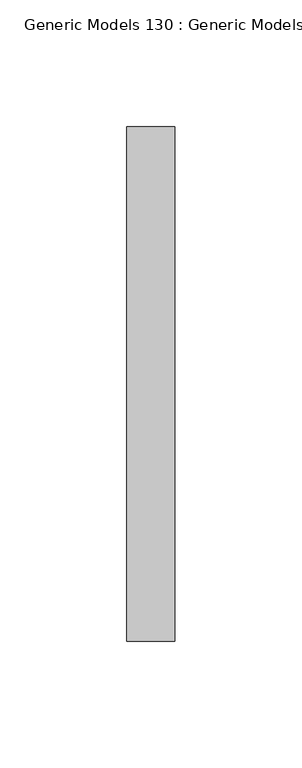
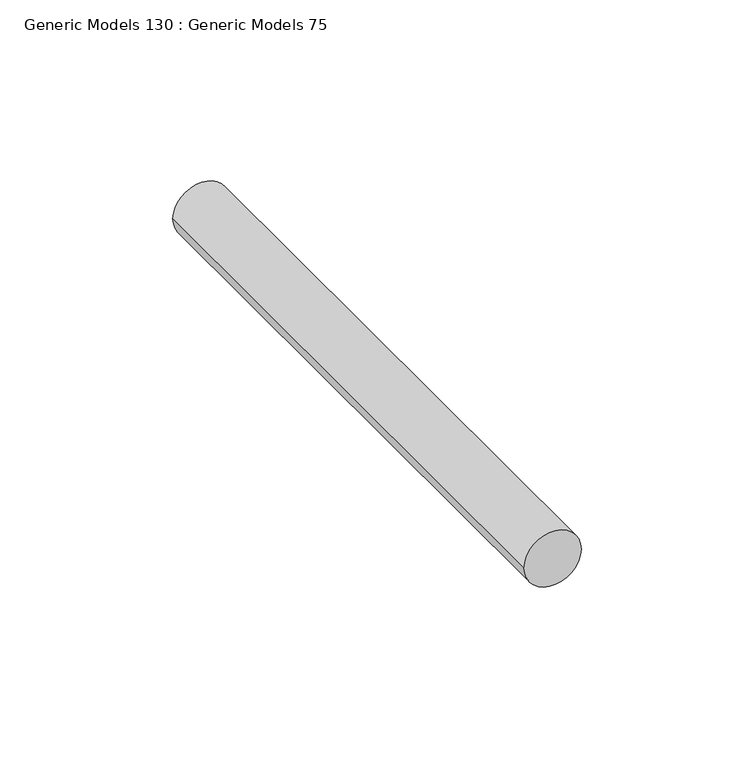
"""IFC4 building model written with IfcOpenShell, lengths in millimetres: proxy geometry, Generic Models 130 : Generic Models 75."""

from ifc_helpers import new_model, si_unit, point, frame, frame_2d, origin, place, context, project, spatial, circle_curve, trimmed, segment, composite_curve, outline, extrude, source, transform, mapped, element, save


def generic_models_130_generic_models_75_e1c93d45(model_context):
    return source(origin(), model_context, "Body", "SweptSolid", [
        extrude(outline(composite_curve([segment(trimmed(circle_curve(frame_2d((268495.4625, 31975.4096032)), 9.525), [point((268495.4625, 31965.8846032))], [point((268495.4625, 31984.9346032))], False, "CARTESIAN"), True, "CONTINUOUS"), segment(trimmed(circle_curve(frame_2d((268495.4625, 31975.4096032)), 9.525), [point((268495.4625, 31984.9346032))], [point((268495.4625, 31965.8846032))], False, "CARTESIAN"), True, "CONTINUOUS")], self_intersect=False)), frame((0.0, 33973.9898424, 0.0), z_axis=(0.0, 1.0, 0.0), x_axis=(0.0, 0.0, 1.0)), (0.0, 0.0, 1.0), 203.2),
    ])


if __name__ == "__main__":
    model = new_model("IFC4")
    model_context = context("Model", 3, world=origin())
    ifc_project = project(units=[si_unit("LENGTHUNIT", "METRE", prefix="MILLI")], contexts=[model_context])
    site = spatial("IfcSite", under=ifc_project)
    building = spatial("IfcBuilding", under=site)
    placement = place(None, origin())
    generic_models_130_generic_models_75_shape = generic_models_130_generic_models_75_e1c93d45(model_context)
    element("IfcBuildingElementProxy", 1, Name="Generic Models 130 : Generic Models 75", ObjectType="Generic Models 130 : Generic Models 75", at=placement, inside=building, context=model_context, shape_type="MappedRepresentation", body=[
        mapped(generic_models_130_generic_models_75_shape, transform((0.0, 0.0, 0.0), x_axis=(1.0, 0.0, 0.0), y_axis=(0.0, 1.0, 0.0), z_axis=(0.0, 0.0, 1.0))),
    ])
    save(model, "model.ifc")
